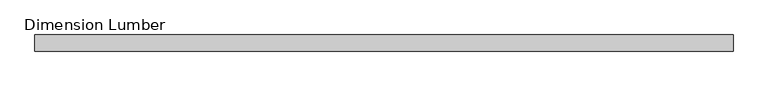
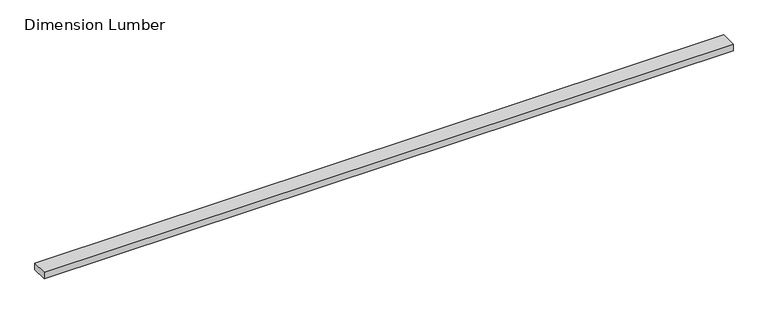
"""IFC4 building model written with IfcOpenShell, lengths in millimetres: beam geometry, Dimension Lumber : Top Supporting Lumbers."""

from ifc_helpers import new_model, si_unit, frame, origin, place, context, project, spatial, polyline, outline, extrude, source, transform, mapped, element, save


def dimension_lumber_1b552245(model_context):
    return source(origin(), model_context, "Body", "SweptSolid", [
        extrude(outline(polyline([(1918.49375, 44.45), (1918.49375, -44.45), (-1918.49375, -44.45), (-1918.49375, 44.45), (1918.49375, 44.45)])), frame((0.0, 0.0, -19.05), z_axis=(0.0, 0.0, 1.0), x_axis=(1.0, 0.0, 0.0)), (0.0, 0.0, 1.0), 38.1),
    ])


if __name__ == "__main__":
    model = new_model("IFC4")
    model_context = context("Model", 3, world=origin())
    ifc_project = project(units=[si_unit("LENGTHUNIT", "METRE", prefix="MILLI")], contexts=[model_context])
    site = spatial("IfcSite", under=ifc_project)
    building = spatial("IfcBuilding", under=site)
    placement = place(None, origin())
    dimension_lumber_shape = dimension_lumber_1b552245(model_context)
    element("IfcBeam", 1, ObjectType="Dimension Lumber : Top Supporting Lumbers", at=placement, inside=building, context=model_context, shape_type="MappedRepresentation", body=[
        mapped(dimension_lumber_shape, transform((0.0, 0.0, 0.0), x_axis=(1.0, 0.0, 0.0), y_axis=(0.0, 1.0, 0.0), z_axis=(0.0, 0.0, 1.0))),
    ])
    save(model, "model.ifc")

# Revit data of these elements
# Type "Dimension Lumber : Top Supporting Lumbers"
#   Assembly Code = "B10"
#   A = 0.0364583 SF
#   Length [instance default] = 5' - 0"
#   b = 0' - 3 1/2"
#   d = 0' - 1 1/2"
#   Structural Material [instance default] = Softwood, Lumber
# Element 1 (IfcBeam, "Dimension Lumber : Top Supporting Lumbers")
#   Structural Material = Douglas Fir #2
#   Materials on its faces: "Douglas Fir #2"
# Materials
#   "Softwood, Lumber": class "Wood", colour RGB 223 192 134, transparency 0, Description = "Pinus Echinata", Cost = 0
#   "Douglas Fir #2": class "Wood", colour RGB 223 192 134, transparency 0, Description = "Pinus Echinata", Cost = 0
